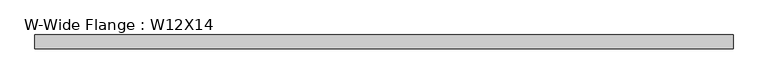
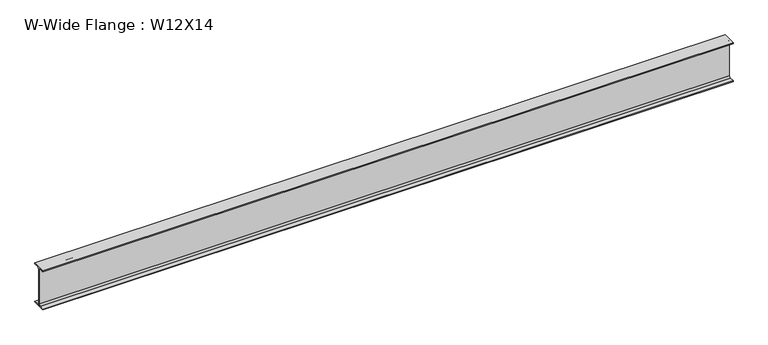
"""IFC4 building model written with IfcOpenShell, lengths in millimetres: beam geometry, W-Wide Flange : W12X14."""

from ifc_helpers import new_model, si_unit, point, frame, frame_2d, origin, place, context, project, spatial, polyline, circle_curve, trimmed, segment, composite_curve, outline, extrude, source, transform, mapped, element, save


def w_wide_flange_w12x14_94fda763(model_context):
    return source(origin(), model_context, "Body", "SweptSolid", [
        extrude(outline(composite_curve([segment(polyline([(50.419, -145.415), (50.419, -151.13), (-50.419, -151.13), (-50.419, -145.415), (-15.875, -145.415)]), True, "CONTINUOUS"), segment(trimmed(circle_curve(frame_2d((-15.875, -132.08)), 13.335), [point((-15.875, -145.415))], [point((-2.54, -132.08))], True, "CARTESIAN"), True, "CONTINUOUS"), segment(polyline([(-2.54, -132.08), (-2.54, 132.08)]), True, "CONTINUOUS"), segment(trimmed(circle_curve(frame_2d((-15.875, 132.08)), 13.335), [point((-2.54, 132.08))], [point((-15.875, 145.415))], True, "CARTESIAN"), True, "CONTINUOUS"), segment(polyline([(-15.875, 145.415), (-50.419, 145.415), (-50.419, 151.13), (50.419, 151.13), (50.419, 145.415), (15.875, 145.415)]), True, "CONTINUOUS"), segment(trimmed(circle_curve(frame_2d((15.875, 132.08)), 13.335), [point((15.875, 145.415))], [point((2.54, 132.08))], True, "CARTESIAN"), True, "CONTINUOUS"), segment(polyline([(2.54, 132.08), (2.54, -132.08)]), True, "CONTINUOUS"), segment(trimmed(circle_curve(frame_2d((15.875, -132.08)), 13.335), [point((2.54, -132.08))], [point((15.875, -145.415))], True, "CARTESIAN"), True, "CONTINUOUS"), segment(polyline([(15.875, -145.415), (50.419, -145.415)]), True, "CONTINUOUS")], self_intersect=False)), frame((-2535.2375, 0.0, 0.0), z_axis=(1.0, 0.0, 0.0), x_axis=(0.0, 1.0, 0.0)), (0.0, 0.0, 1.0), 5070.475),
    ])


if __name__ == "__main__":
    model = new_model("IFC4")
    model_context = context("Model", 3, world=origin())
    ifc_project = project(units=[si_unit("LENGTHUNIT", "METRE", prefix="MILLI")], contexts=[model_context])
    site = spatial("IfcSite", under=ifc_project)
    building = spatial("IfcBuilding", under=site)
    placement = place(None, origin())
    w_wide_flange_w12x14_shape = w_wide_flange_w12x14_94fda763(model_context)
    element("IfcBeam", 1, ObjectType="W-Wide Flange : W12X14", at=placement, inside=building, context=model_context, shape_type="MappedRepresentation", body=[
        mapped(w_wide_flange_w12x14_shape, transform((0.0, 0.0, 0.0), x_axis=(1.0, 0.0, 0.0), y_axis=(0.0, 1.0, 0.0), z_axis=(0.0, 0.0, 1.0))),
    ])
    save(model, "model.ifc")

# Revit data of these elements
# Type "W-Wide Flange : W12X14"
#   Assembly Code = "B10"
#   W = 14
#   Length [instance default] = 1524 mm
#   bf = 100.838 mm
#   d = 302.26 mm
#   k = 19.05 mm
#   k2 = 13.335 mm
#   tf = 5.715 mm
#   tw = 5.08 mm
#   A = 0.00268387 m²
#   Structural Material [instance default] = Steel ASTM A992
# Element 1 (IfcBeam, "W-Wide Flange : W12X14")
#   Structural Material = Aluminum, Anodized Red
#   Materials on its faces: "Aluminum, Anodized Red"
# Materials
#   "Steel ASTM A992": class "Metal", colour RGB 128 0 0, transparency 0, Description = "Structural steel 50ksi", Cost = 0
#   "Aluminum, Anodized Red": class "Metal", colour RGB 120 120 120, transparency 0, Description = "Anodized aluminum, red", Cost = 0
